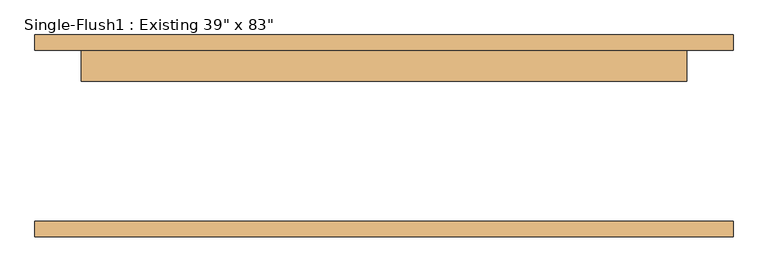
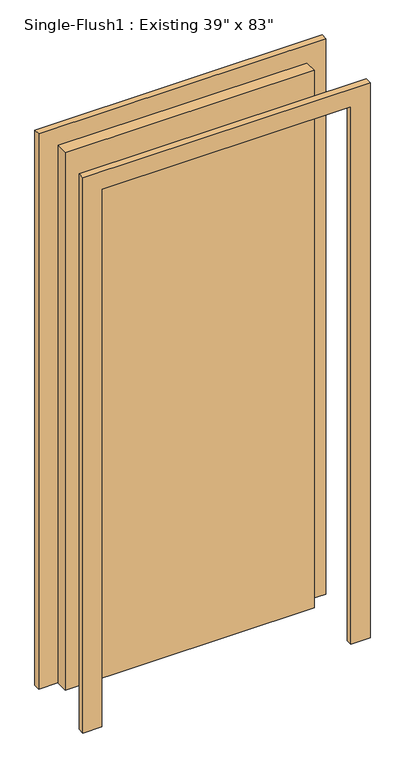
"""IFC4 building model written with IfcOpenShell, lengths in millimetres: door geometry."""

from ifc_helpers import new_model, si_unit, frame, origin, origin_with_axes, place, context, project, spatial, polyline, outline, extrude, source, transform, mapped, element, save


def door_3f262015(model_context):
    return source(origin(), model_context, "Body", "SweptSolid", [
        extrude(outline(polyline([(2336.8, -571.5), (0.0, -571.5), (0.0, -495.3), (2260.6, -495.3), (2260.6, 495.3), (0.0, 495.3), (0.0, 571.5), (2336.8, 571.5), (2336.8, -571.5)])), frame((0.0, 139.7, 0.0), z_axis=(0.0, 1.0, 0.0), x_axis=(0.0, 0.0, 1.0)), (0.0, 0.0, 1.0), 25.4),
        extrude(outline(polyline([(2336.8, 571.5), (2336.8, -571.5), (0.0, -571.5), (0.0, -495.3), (2260.6, -495.3), (2260.6, 495.3), (0.0, 495.3), (0.0, 571.5), (2336.8, 571.5)])), frame((0.0, -165.1, 0.0), z_axis=(0.0, 1.0, 0.0), x_axis=(0.0, 0.0, 1.0)), (0.0, 0.0, 1.0), 25.4),
        extrude(outline(polyline([(495.3, 88.9), (-495.3, 88.9), (-495.3, 139.7), (495.3, 139.7), (495.3, 88.9)])), origin_with_axes(), (0.0, 0.0, 1.0), 2260.6),
    ])


if __name__ == "__main__":
    model = new_model("IFC4")
    model_context = context("Model", 3, world=origin())
    ifc_project = project(units=[si_unit("LENGTHUNIT", "METRE", prefix="MILLI")], contexts=[model_context])
    site = spatial("IfcSite", under=ifc_project)
    building = spatial("IfcBuilding", under=site)
    placement = place(None, origin())
    door_shape = door_3f262015(model_context)
    element("IfcDoor", 1, ObjectType="Single-Flush1 : Existing 39\" x 83\"", at=placement, inside=building, context=model_context, shape_type="MappedRepresentation", body=[
        mapped(door_shape, transform((0.0, 0.0, 0.0), x_axis=(1.0, 0.0, 0.0), y_axis=(0.0, 1.0, 0.0), z_axis=(0.0, 0.0, 1.0))),
    ])
    save(model, "model.ifc")

# Revit data of these elements
# Type "Single-Flush1 : Existing 39\" x 83\""
#   Type Mark = "EX"
#   Construction Type Id = "MDOOR"
#   Assembly Code = "C1020"
#   Analytic Construction = "Metal"
#   Thickness = 0' - 2"
#   Heat Transfer Coefficient (U) = 3.7021 W/(m²·K)
#   Height = 7' - 5"
#   Trim Projection Ext = 0' - 1"
#   Trim Projection Int = 0' - 1"
#   Trim Width = 0' - 3"
#   Width = 3' - 3"
#   Door Material = Door - Panel
#   Frame Material = Door - Frame
#   Visual Light Transmittance = 0
#   Solar Heat Gain Coefficient = 0
#   Function = (empty or 0)
#   Wall Closure = (empty or 0)
# Element 1 (IfcDoor, "Single-Flush1 : Existing 39\" x 83\"")
#   Materials on its faces: "Door - Frame", "Door - Panel"
# Materials
#   "Door - Panel": class "Wood", colour RGB 255 255 255, transparency 0, Cost = 0
#   "Door - Frame": class "Miscellaneous", colour RGB 255 255 255, transparency 0, Cost = 0
